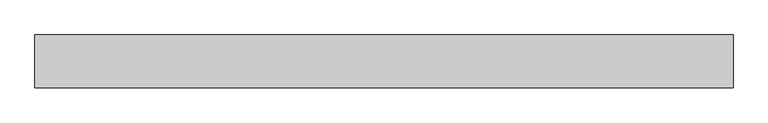
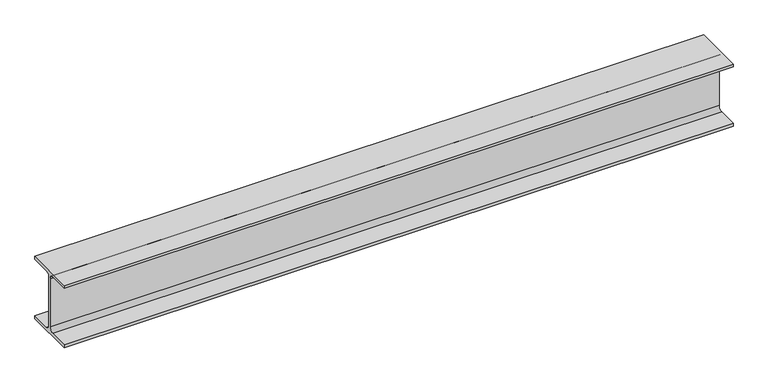
"""IFC4 building model written with IfcOpenShell, lengths in millimetres: beam geometry, 0912_Steel Framing_H-KSD3502 : H_SB_ASB_H-194x150x6x9."""

from ifc_helpers import new_model, si_unit, point, frame, frame_2d, origin, place, context, project, spatial, polyline, circle_curve, trimmed, segment, composite_curve, outline, extrude, source, transform, mapped, element, save


def beam_eef1affa(model_context):
    return source(origin(), model_context, "Body", "SweptSolid", [
        extrude(outline(composite_curve([segment(polyline([(75.0, -88.0), (75.0, -97.0), (-75.0, -97.0), (-75.0, -88.0), (-16.0, -88.0)]), True, "CONTINUOUS"), segment(trimmed(circle_curve(frame_2d((-16.0, -75.0)), 13.0), [point((-16.0, -88.0))], [point((-3.0, -75.0))], True, "CARTESIAN"), True, "CONTINUOUS"), segment(polyline([(-3.0, -75.0), (-3.0, 75.0)]), True, "CONTINUOUS"), segment(trimmed(circle_curve(frame_2d((-16.0, 75.0)), 13.0), [point((-3.0, 75.0))], [point((-16.0, 88.0))], True, "CARTESIAN"), True, "CONTINUOUS"), segment(polyline([(-16.0, 88.0), (-75.0, 88.0), (-75.0, 97.0), (75.0, 97.0), (75.0, 88.0), (16.0, 88.0)]), True, "CONTINUOUS"), segment(trimmed(circle_curve(frame_2d((16.0, 75.0)), 13.0), [point((16.0, 88.0))], [point((3.0, 75.0))], True, "CARTESIAN"), True, "CONTINUOUS"), segment(polyline([(3.0, 75.0), (3.0, -75.0)]), True, "CONTINUOUS"), segment(trimmed(circle_curve(frame_2d((16.0, -75.0)), 13.0), [point((3.0, -75.0))], [point((16.0, -88.0))], True, "CARTESIAN"), True, "CONTINUOUS"), segment(polyline([(16.0, -88.0), (75.0, -88.0)]), True, "CONTINUOUS")], self_intersect=False)), frame((-988.3546085, 0.0, 0.0), z_axis=(1.0, 0.0, 0.0), x_axis=(0.0, 1.0, 0.0)), (0.0, 0.0, 1.0), 1976.709217),
    ])


if __name__ == "__main__":
    model = new_model("IFC4")
    model_context = context("Model", 3, world=origin())
    ifc_project = project(units=[si_unit("LENGTHUNIT", "METRE", prefix="MILLI")], contexts=[model_context])
    site = spatial("IfcSite", under=ifc_project)
    building = spatial("IfcBuilding", under=site)
    placement = place(None, origin())
    beam_shape = beam_eef1affa(model_context)
    element("IfcBeam", 1, ObjectType="0912_Steel Framing_H-KSD3502 : H_SB_ASB_H-194x150x6x9", at=placement, inside=building, context=model_context, shape_type="MappedRepresentation", body=[
        mapped(beam_shape, transform((0.0, 0.0, 0.0), x_axis=(1.0, 0.0, 0.0), y_axis=(0.0, 1.0, 0.0), z_axis=(0.0, 0.0, 1.0))),
    ])
    save(model, "model.ifc")

# Revit data of these elements
# Type "0912_Steel Framing_H-KSD3502 : H_SB_ASB_H-194x150x6x9"
#   H_WM Code_1 = "S01AA002-00001 | Main Steel Structure Fabrication Work | Shelter/Building | Medium Steel - Standard (90KG/M>Weight≥30KG/M) | Material: (   )"
#   H_WM Code_2 = "S03AA028-00001 | Main Steel Structure Erection Work | Shelter/Building | Medium Steel (90KG/M>Weight≥30KG/M) | Material: (   )"
#   H_WM Code_3 = "S01AA010-00001 | Main Steel Structure Fabrication Work | Shelter/Building | Steel Painting/Coating | for Non-Fireproofed Steel Surface, Surface Preparation, Primer, Second & Final Coat | Material: (   )"
#   H_Q'ty Cal Type Tag = "SB-Q2"
#   Width = 15.0 cm
#   Web Thickness = 0.6 cm
#   Web Fillet = 1.3 cm
#   Warping Constant = 43316.0 cm⁶
#   W = 0
#   Torsional Moment of Inertia = 8.622 cm⁴
#   Section Area = 39.01 cm²
#   Plastic Modulus weak axis = 104.0 cm³
#   Plastic Modulus strong axis = 309.0 cm³
#   Perimeter = 0.95 m²/m
#   Nominal Weight = 30.60 kgf/m
#   Moment of Inertia weak axis = 507.00 cm⁴
#   Moment of Inertia strong axis = 2690.00 cm⁴
#   Height = 19.4 cm
#   Flange Thickness = 0.9 cm
#   Elastic Modulus weak axis = 67.6 cm³
#   Elastic Modulus strong axis = 277.0 cm³
#   Centroid Vertical = 9.7 cm
#   Centroid Horizontal = 7.5 cm
#   Ix = 26900000
#   Length [instance default] = 1.5240 m
#   Zx = 309000
#   b = 0.1500 m
#   h = 0.1940 m
#   r = 0.0130 m
#   s = 0.0060 m
#   t = 0.0090 m
#   A = 0.003901 m²
#   Structural Material [instance default] = Steel, 45-345
#   Assembly Code = ""
# Element 1 (IfcBeam, "0912_Steel Framing_H-KSD3502 : H_SB_ASB_H-194x150x6x9")
#   Structural Material = none
# Materials
#   "Steel, 45-345": class "Metal", colour RGB 189 187 185, transparency 0, Description = "Steel 345 MPa", Cost = 0
